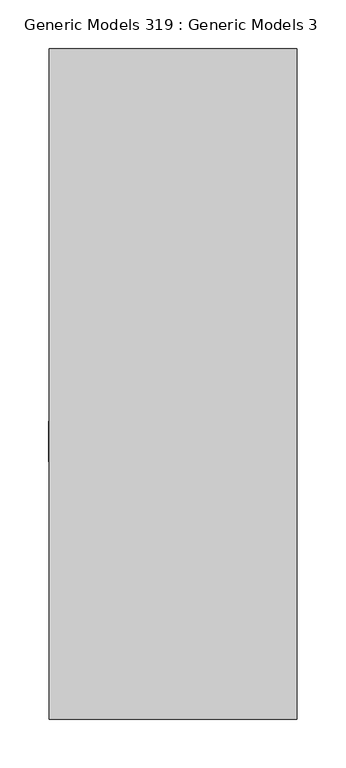
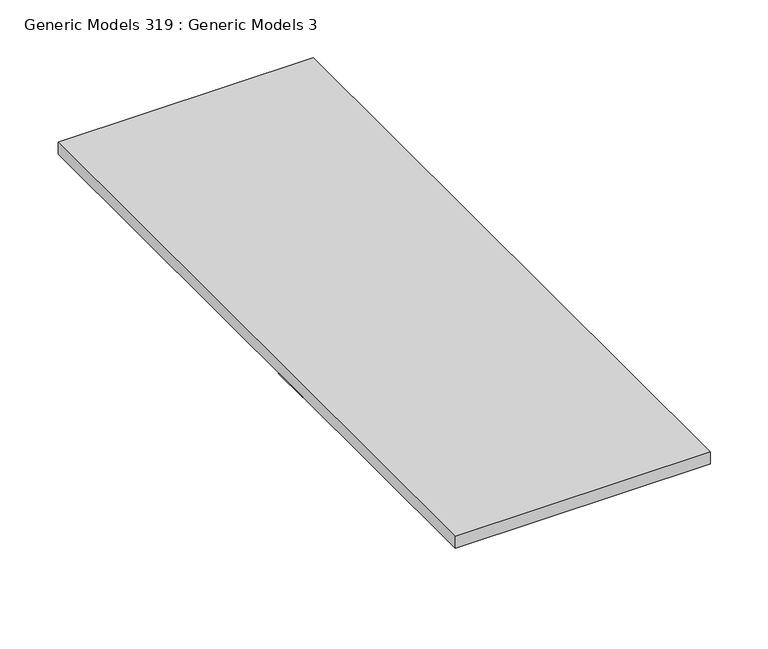
"""IFC4 building model written with IfcOpenShell, lengths in millimetres: proxy geometry, Generic Models 319 : Generic Models 3."""

import ifcopenshell
import ifcopenshell.guid

model = None  # the IFC model being written
_history = None  # IfcOwnerHistory: only IFC2X3 demands one
_inside = {}  # id of a spatial element -> (the spatial element, [elements in it])
_under = {}  # id of a project, library or spatial element -> (it, [spatial elements below it])
_declared = {}  # id of a project -> (the project, [libraries it declares])
_typed = {}  # id of a type object -> (the type object, [elements of that type])
_made_of = {}  # id of a material, layer set ... -> (it, [elements and type objects made of it])


def new_model(schema):
    """Start an empty IFC model of exactly this schema.

    Asked for "IFC4X3", IfcOpenShell would pick the latest addendum, in which some entities
    have other attributes; the version numbers below select the first issue.
    IFC2X3 requires an IfcOwnerHistory on every rooted entity: one is made here for all.
    """
    global model, _history
    if schema == "IFC4X3":
        model = ifcopenshell.file(schema_version=(4, 3, 0, 0))
    else:
        model = ifcopenshell.file(schema=schema)
    _inside.clear()
    _under.clear()
    _declared.clear()
    _typed.clear()
    _made_of.clear()
    _history = None
    if model.schema == "IFC2X3":
        org = make("IfcOrganization", Name="unknown")
        user = make(
            "IfcPersonAndOrganization",
            ThePerson=make("IfcPerson", FamilyName="unknown"),
            TheOrganization=org,
        )
        app = make(
            "IfcApplication",
            ApplicationDeveloper=org,
            Version="unknown",
            ApplicationFullName="unknown",
            ApplicationIdentifier="unknown",
        )
        _history = make(
            "IfcOwnerHistory",
            OwningUser=user,
            OwningApplication=app,
            ChangeAction="ADDED",
            CreationDate=0,
        )
    return model


def make(cls, **values):
    """One entity of the class cls with the attributes given. An attribute that is None is left unset."""
    return model.create_entity(
        cls, **{name: value for name, value in values.items() if value is not None}
    )


def rooted(cls, **values):
    """An entity with a GlobalId (a new one), such as an element, a storey or a relation."""
    return make(cls, GlobalId=ifcopenshell.guid.new(), OwnerHistory=_history, **values)


def si_unit(unit_type, name, prefix=None):
    """IfcSIUnit, for example si_unit("LENGTHUNIT", "METRE", prefix="MILLI")."""
    return make("IfcSIUnit", UnitType=unit_type, Prefix=prefix, Name=name)


def assignment(units):
    """IfcUnitAssignment: the units of a project."""
    return None if units is None else make("IfcUnitAssignment", Units=units)


def point(xyz):
    """IfcCartesianPoint."""
    return None if xyz is None else make("IfcCartesianPoint", Coordinates=xyz)


def direction(xyz):
    """IfcDirection."""
    return None if xyz is None else make("IfcDirection", DirectionRatios=xyz)


def frame(location, z_axis=None, x_axis=None):
    """IfcAxis2Placement3D, a coordinate frame: its origin and axes. An axis left out is left unset."""
    return make(
        "IfcAxis2Placement3D",
        Location=point(location),
        Axis=direction(z_axis),
        RefDirection=direction(x_axis),
    )


def origin():
    """The frame at (0, 0, 0) with its axes left unset."""
    return frame((0.0, 0.0, 0.0))


def place(relative_to, where):
    """IfcLocalPlacement: puts the frame where relative to a parent placement (None: the world)."""
    return make(
        "IfcLocalPlacement", PlacementRelTo=relative_to, RelativePlacement=where
    )


def context(
    kind, dimensions, precision=None, world=None, true_north=None, identifier=None
):
    """IfcGeometricRepresentationContext, for example the 3D "Model" context."""
    return make(
        "IfcGeometricRepresentationContext",
        ContextIdentifier=identifier,
        ContextType=kind,
        CoordinateSpaceDimension=dimensions,
        Precision=precision,
        WorldCoordinateSystem=world,
        TrueNorth=true_north,
    )


def project(units=None, contexts=None):
    """IfcProject with its units and contexts."""
    return rooted(
        "IfcProject",
        Name="project",
        RepresentationContexts=contexts,
        UnitsInContext=assignment(units),
    )


def spatial(cls, under=None, at=None, **own):
    """A site, building, storey or space (cls), placed at a placement, below another one or the project."""
    s = rooted(cls, ObjectPlacement=at, **own)
    if under is not None:
        _under.setdefault(under.id(), (under, []))[1].append(s)
    return s


def polyline(points):
    """IfcPolyline through the points."""
    return make("IfcPolyline", Points=[point(p) for p in points])


def outline(outer, holes=None, kind="AREA"):
    """IfcArbitraryClosedProfileDef: a profile drawn as a closed curve; with holes, ...WithVoids."""
    if holes is None:
        return make("IfcArbitraryClosedProfileDef", ProfileType=kind, OuterCurve=outer)
    return make(
        "IfcArbitraryProfileDefWithVoids",
        ProfileType=kind,
        OuterCurve=outer,
        InnerCurves=holes,
    )


def extrude(swept, where, along, depth):
    """IfcExtrudedAreaSolid: the profile swept, set in the frame where, extruded along a direction by depth."""
    return make(
        "IfcExtrudedAreaSolid",
        SweptArea=swept,
        Position=where,
        ExtrudedDirection=direction(along),
        Depth=depth,
    )


def shape(context_of_items, identifier, shape_type, items):
    """IfcShapeRepresentation: the items that make up one representation, for example the "Body"."""
    return make(
        "IfcShapeRepresentation",
        ContextOfItems=context_of_items,
        RepresentationIdentifier=identifier,
        RepresentationType=shape_type,
        Items=items,
    )


def source(mapping_origin, context_of_items, identifier, shape_type, items):
    """IfcRepresentationMap: a shape defined once, which mapped items show again and again."""
    return make(
        "IfcRepresentationMap",
        MappingOrigin=mapping_origin,
        MappedRepresentation=shape(context_of_items, identifier, shape_type, items),
    )


def transform(
    local_origin,
    x_axis=None,
    y_axis=None,
    z_axis=None,
    scale=None,
    scale2=None,
    scale3=None,
    uniform=True,
):
    """IfcCartesianTransformationOperator3D, or its non-uniform kind. x_axis, y_axis, z_axis: its Axis1, 2, 3."""
    if uniform:
        return make(
            "IfcCartesianTransformationOperator3D",
            Axis1=direction(x_axis),
            Axis2=direction(y_axis),
            LocalOrigin=point(local_origin),
            Scale=scale,
            Axis3=direction(z_axis),
        )
    return make(
        "IfcCartesianTransformationOperator3DnonUniform",
        Axis1=direction(x_axis),
        Axis2=direction(y_axis),
        LocalOrigin=point(local_origin),
        Scale=scale,
        Axis3=direction(z_axis),
        Scale2=scale2,
        Scale3=scale3,
    )


def mapped(mapping_source, mapping_target):
    """IfcMappedItem: shows the shape of a source again, moved by a transform."""
    return make(
        "IfcMappedItem", MappingSource=mapping_source, MappingTarget=mapping_target
    )


def made_of(thing, what):
    """Note that an element or type object is made of a material, layer set ...; save() writes the relation."""
    if what is not None:
        _made_of.setdefault(what.id(), (what, []))[1].append(thing)
    return thing


def element(
    cls,
    number,
    at=None,
    inside=None,
    cuts=None,
    type_object=None,
    material=None,
    context=None,
    identifier="Body",
    shape_type=None,
    held_by="IfcProductDefinitionShape",
    body=None,
    shapes=None,
    **own,
):
    """One element of the class cls, such as IfcWall. Its Tag is "e" and its number.

    at: its placement. inside: the storey or other place that contains it. cuts: it is an
    opening in that element (IfcRelVoidsElement). A single representation is given by context,
    identifier, shape_type and body (its items); several are given by shapes. held_by: the class
    of the entity that holds the representations. save() writes the other relations.
    """
    e = rooted(cls, Tag="e%d" % number, ObjectPlacement=at, **own)
    if body is not None:
        shapes = [shape(context, identifier, shape_type, body)]
    if shapes is not None:
        e.Representation = make(held_by, Representations=shapes)
    if inside is not None:
        _inside.setdefault(inside.id(), (inside, []))[1].append(e)
    if cuts is not None:
        rooted(
            "IfcRelVoidsElement", RelatingBuildingElement=cuts, RelatedOpeningElement=e
        )
    if type_object is not None:
        _typed.setdefault(type_object.id(), (type_object, []))[1].append(e)
    return made_of(e, material)


def aggregate(whole, parts):
    """IfcRelAggregates: a whole, such as a stair, and the parts it consists of."""
    return rooted("IfcRelAggregates", RelatingObject=whole, RelatedObjects=parts)


def save(model, path):
    """Write the relations noted so far, then the file.

    IfcRelAggregates (storeys below a building ...), IfcRelContainedInSpatialStructure (elements
    in a storey), IfcRelDefinesByType, IfcRelAssociatesMaterial and IfcRelDeclares: one each for
    every whole, place, type object, material and project.
    """
    for whole, parts in _under.values():
        aggregate(whole, parts)
    for where, things in _inside.values():
        rooted(
            "IfcRelContainedInSpatialStructure",
            RelatedElements=things,
            RelatingStructure=where,
        )
    for kind, things in _typed.values():
        rooted("IfcRelDefinesByType", RelatedObjects=things, RelatingType=kind)
    for what, things in _made_of.values():
        rooted("IfcRelAssociatesMaterial", RelatedObjects=things, RelatingMaterial=what)
    for by, libraries in _declared.values():
        rooted("IfcRelDeclares", RelatingContext=by, RelatedDefinitions=libraries)
    model.write(path)


def generic_models_319_generic_models_3_f40ae0e6(model_context):
    return source(origin(), model_context, "Body", "SweptSolid", [
        extrude(outline(polyline([(124453.396, 2958.6524467), (124408.4947194, 3003.5537273), (124408.4947194, 3150.7703783), (124440.538773, 3209.5498486), (124453.396, 3209.5498486), (124453.396, 2958.6524467)])), frame((0.0, 662.7539193, 0.0), z_axis=(0.0, 1.0, 0.0), x_axis=(0.0, 0.0, 1.0)), (0.0, 0.0, 1.0), 41.7770469),
        extrude(outline(polyline([(2958.9263704, 1085.2769662), (3212.9263704, 1085.2769662), (3212.9263704, 399.7309662), (2958.9263704, 399.7309662), (2958.9263704, 1085.2769662)])), frame((0.0, 0.0, 124453.396), z_axis=(0.0, 0.0, 1.0), x_axis=(1.0, 0.0, 0.0)), (0.0, 0.0, 1.0), 12.7),
    ])


if __name__ == "__main__":
    model = new_model("IFC4")
    model_context = context("Model", 3, world=origin())
    ifc_project = project(units=[si_unit("LENGTHUNIT", "METRE", prefix="MILLI")], contexts=[model_context])
    site = spatial("IfcSite", under=ifc_project)
    building = spatial("IfcBuilding", under=site)
    placement = place(None, origin())
    generic_models_319_generic_models_3_shape = generic_models_319_generic_models_3_f40ae0e6(model_context)
    element("IfcBuildingElementProxy", 1, Name="Generic Models 319 : Generic Models 3", ObjectType="Generic Models 319 : Generic Models 3", at=placement, inside=building, context=model_context, shape_type="MappedRepresentation", body=[
        mapped(generic_models_319_generic_models_3_shape, transform((0.0, 0.0, 0.0), x_axis=(1.0, 0.0, 0.0), y_axis=(0.0, 1.0, 0.0), z_axis=(0.0, 0.0, 1.0))),
    ])
    save(model, "model.ifc")

# Revit data of these elements
# Element 1 (IfcBuildingElementProxy, "Generic Models 319 : Generic Models 3")
#   Materials on its faces: "_SHAPED \"T\" TREAD SUPPORT PER STRUCTURAL, PAINTED"
# Materials
#   "_SHAPED \"T\" TREAD SUPPORT PER STRUCTURAL, PAINTED": class "Metal", colour RGB 199 199 199, transparency 0, Description = "Structural steel 50ksi", Cost = 0
